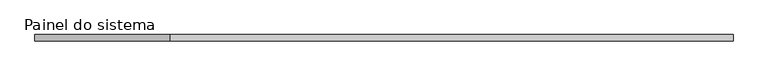
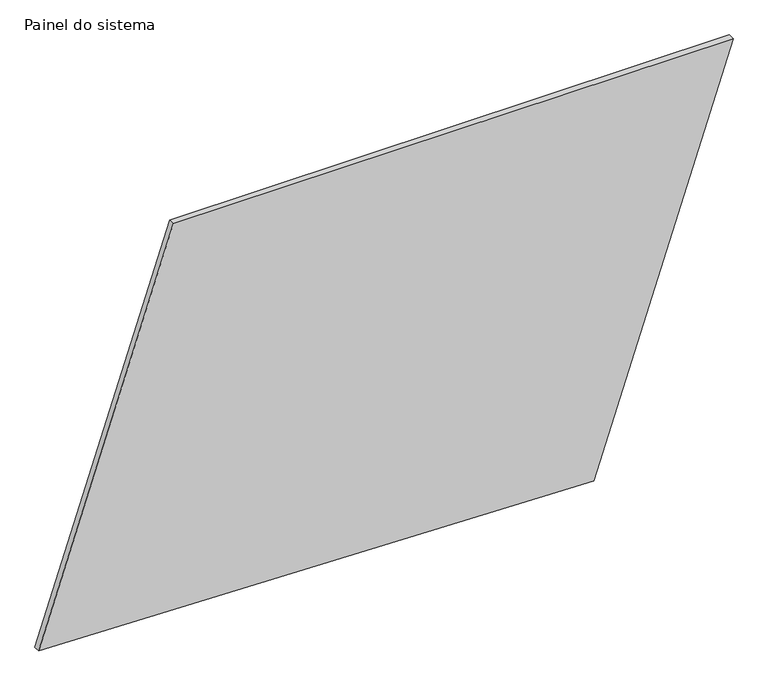
"""IFC4 building model written with IfcOpenShell, lengths in millimetres: plate geometry, Painel do sistema : Envidraçado."""

from ifc_helpers import new_model, si_unit, frame, origin, place, context, project, spatial, polyline, outline, extrude, source, transform, mapped, element, save


def painel_do_sistema_cf0f4c89(model_context):
    return source(origin(), model_context, "Body", "SweptSolid", [
        extrude(outline(polyline([(56.5275925, -1348.0181232), (0.0, 806.2590599), (1627.4644698, 1348.0181232), (1627.4644698, -825.0762667), (56.5275925, -1348.0181232)])), frame((0.0, 24.5, 0.0), z_axis=(0.0, 1.0, 0.0), x_axis=(0.0, 0.0, 1.0)), (0.0, 0.0, 1.0), 25.0),
    ])


if __name__ == "__main__":
    model = new_model("IFC4")
    model_context = context("Model", 3, world=origin())
    ifc_project = project(units=[si_unit("LENGTHUNIT", "METRE", prefix="MILLI")], contexts=[model_context])
    site = spatial("IfcSite", under=ifc_project)
    building = spatial("IfcBuilding", under=site)
    placement = place(None, origin())
    painel_do_sistema_shape = painel_do_sistema_cf0f4c89(model_context)
    element("IfcPlate", 1, ObjectType="Painel do sistema : Envidraçado", at=placement, inside=building, context=model_context, shape_type="MappedRepresentation", body=[
        mapped(painel_do_sistema_shape, transform((0.0, 0.0, 0.0), x_axis=(1.0, 0.0, 0.0), y_axis=(0.0, 1.0, 0.0), z_axis=(0.0, 0.0, 1.0))),
    ])
    save(model, "model.ifc")

# Revit data of these elements
# Type "Painel do sistema : Envidraçado"
#   Construction Type Id = "GSP4R"
#   Analytic Construction = "Vidraça única Pilkington 1/8 pol"
#   Visual Light Transmittance = 0.9
#   Solar Heat Gain Coefficient = 0.86
#   Heat Transfer Coefficient (U) = 6.7069 W/(m²·K)
# Element 1 (IfcPlate, "Painel do sistema : Envidraçado")
#   Materials on its faces: "Vidro"
# Materials
#   "Vidro": class "Vidro", colour RGB 0 128 192, transparency 0.9, Description = "Vidro de sílica", Cost = 0
